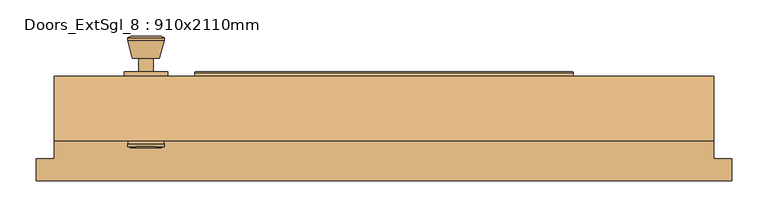
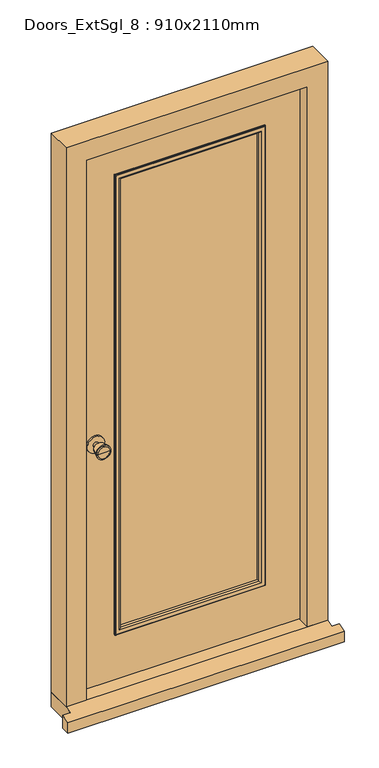
"""IFC4 building model written with IfcOpenShell, lengths in millimetres: door geometry, Doors_ExtSgl_8 : 910x2110mm."""

from ifc_helpers import new_model, si_unit, point, frame, frame_2d, origin, place, context, project, spatial, polyline, circle_curve, ellipse_curve, trimmed, segment, composite_curve, outline, extrude, faceted_brep, source, transform, mapped, element, save
from ifc_brep_helpers import plane_surface, cylinder_surface, revolved_surface, advanced_brep


def doors_extsgl_8_910x2110mm_7df14444(model_context):
    return source(origin(), model_context, "Body", "SolidModel", [
        advanced_brep(
        [(-328.5, -25.0, 950.0), (-338.5, -25.0, 950.0), (-318.5, -25.0, 950.0), (-308.0241324, 24.0, 950.0), (-348.9758676, 24.0, 950.0), (-328.5, 24.0, 950.0), (-303.5, 22.1721319, 950.0), (-353.5, 22.1721319, 950.0), (-303.5, 18.7084537, 950.0), (-353.5, 18.7084537, 950.0), (-309.863764, -6.0, 950.0), (-347.136236, -6.0, 950.0), (-318.5, -6.0, 950.0), (-338.5, -6.0, 950.0)],
        [
            (0, 1),
            (1, 2, circle_curve(frame((-328.5, -25.0, 950.0), z_axis=(0.0, -1.0, 0.0), x_axis=(-1.0, 0.0, 0.0)), 10.0)),
            (2, 0),
            (2, 1, circle_curve(frame((-328.5, -25.0, 950.0), z_axis=(0.0, -1.0, 0.0), x_axis=(-1.0, 0.0, 0.0)), 10.0)),
            (3, 4, circle_curve(frame((-328.5, 24.0, 950.0), z_axis=(0.0, 1.0, 0.0), x_axis=(-1.0, 0.0, 0.0)), 20.4758676)),
            (4, 5),
            (5, 3),
            (4, 3, circle_curve(frame((-328.5, 24.0, 950.0), z_axis=(0.0, 1.0, 0.0), x_axis=(-1.0, 0.0, 0.0)), 20.4758676)),
            (6, 7, circle_curve(frame((-328.5, 22.1721319, 950.0), z_axis=(0.0, 1.0, 0.0), x_axis=(-1.0, 0.0, 0.0)), 25.0)),
            (7, 4),
            (3, 6),
            (7, 6, circle_curve(frame((-328.5, 22.1721319, 950.0), z_axis=(0.0, 1.0, 0.0), x_axis=(-1.0, 0.0, 0.0)), 25.0)),
            (8, 9, circle_curve(frame((-328.5, 18.7084537, 950.0), z_axis=(0.0, 1.0, 0.0), x_axis=(-1.0, 0.0, 0.0)), 25.0)),
            (9, 7),
            (6, 8),
            (9, 8, circle_curve(frame((-328.5, 18.7084537, 950.0), z_axis=(0.0, 1.0, 0.0), x_axis=(-1.0, 0.0, 0.0)), 25.0)),
            (10, 11, circle_curve(frame((-328.5, -6.0, 950.0), z_axis=(0.0, 1.0, 0.0), x_axis=(-1.0, 0.0, 0.0)), 18.636236)),
            (11, 9),
            (8, 10),
            (11, 10, circle_curve(frame((-328.5, -6.0, 950.0), z_axis=(0.0, 1.0, 0.0), x_axis=(-1.0, 0.0, 0.0)), 18.636236)),
            (12, 13, circle_curve(frame((-328.5, -6.0, 950.0), z_axis=(0.0, 1.0, 0.0), x_axis=(-1.0, 0.0, 0.0)), 10.0)),
            (13, 11),
            (10, 12),
            (13, 12, circle_curve(frame((-328.5, -6.0, 950.0), z_axis=(0.0, 1.0, 0.0), x_axis=(-1.0, 0.0, 0.0)), 10.0)),
            (1, 13),
            (12, 2),
        ],
        [
            plane_surface(frame((-328.5, -25.0, 950.0), z_axis=(0.0, -1.0, 0.0), x_axis=(-1.0, 0.0, 0.0))),
            plane_surface(frame((-328.5, 24.0, 950.0), z_axis=(0.0, 1.0, 0.0), x_axis=(-1.0, 0.0, 0.0))),
            revolved_surface(polyline([(-348.9758676, 24.0, 950.0), (-353.5, 22.1721319, 950.0)]), (-328.5, -25.0, 950.0), (0.0, -1.0, 0.0)),
            cylinder_surface(frame((-328.5, -25.0, 950.0), z_axis=(0.0, -1.0, 0.0), x_axis=(-1.0, 0.0, 0.0)), 25.0),
            revolved_surface(polyline([(-353.5, 18.7084537, 950.0), (-347.136236, -6.0, 950.0)]), (-328.5, -25.0, 950.0), (0.0, -1.0, 0.0)),
            plane_surface(frame((-328.5, -6.0, 950.0), z_axis=(0.0, -1.0, 0.0), x_axis=(-1.0, 0.0, 0.0))),
            cylinder_surface(frame((-328.5, -25.0, 950.0), z_axis=(0.0, -1.0, 0.0), x_axis=(-1.0, 0.0, 0.0)), 10.0),
        ],
        [
            (0, [[1, 2, 3]]),
            (0, [[-3, 4, -1]]),
            (1, [[5, 6, 7]]),
            (1, [[8, -7, -6]]),
            (2, [[9, 10, -5, 11]]),
            (2, [[12, -11, -8, -10]]),
            (3, [[13, 14, -9, 15]]),
            (3, [[16, -15, -12, -14]]),
            (4, [[17, 18, -13, 19]]),
            (4, [[20, -19, -16, -18]]),
            (5, [[21, 22, -17, 23]]),
            (5, [[24, -23, -20, -22]]),
            (6, [[-2, 25, -21, 26]]),
            (6, [[-4, -26, -24, -25]]),
        ],
    ),
        extrude(outline(composite_curve([segment(trimmed(circle_curve(frame_2d((950.0, -328.5)), 30.0), [point((950.0, -358.5))], [point((950.0, -298.5))], False, "CARTESIAN"), True, "CONTINUOUS"), segment(trimmed(circle_curve(frame_2d((950.0, -328.5)), 30.0), [point((950.0, -298.5))], [point((950.0, -358.5))], False, "CARTESIAN"), True, "CONTINUOUS")], self_intersect=False)), frame((0.0, -31.0, 0.0), z_axis=(0.0, 1.0, 0.0), x_axis=(0.0, 0.0, 1.0)), (0.0, 0.0, 1.0), 6.0),
        advanced_brep(
        [(-328.5, -81.0, 950.0), (-318.5, -81.0, 950.0), (-338.5, -81.0, 950.0), (-308.0241324, -130.0, 950.0), (-328.5, -130.0, 950.0), (-348.9758676, -130.0, 950.0), (-303.5, -128.1721319, 950.0), (-353.5, -128.1721319, 950.0), (-303.5, -124.7084537, 950.0), (-353.5, -124.7084537, 950.0), (-309.863764, -100.0, 950.0), (-347.136236, -100.0, 950.0), (-318.5, -100.0, 950.0), (-338.5, -100.0, 950.0)],
        [
            (0, 1),
            (1, 2, circle_curve(frame((-328.5, -81.0, 950.0), z_axis=(0.0, 1.0, 0.0), x_axis=(-1.0, 0.0, 0.0)), 10.0)),
            (2, 0),
            (2, 1, circle_curve(frame((-328.5, -81.0, 950.0), z_axis=(0.0, 1.0, 0.0), x_axis=(-1.0, 0.0, 0.0)), 10.0)),
            (3, 4),
            (4, 5),
            (5, 3, circle_curve(frame((-328.5, -130.0, 950.0), z_axis=(0.0, -1.0, 0.0), x_axis=(-1.0, 0.0, 0.0)), 20.4758676)),
            (3, 5, circle_curve(frame((-328.5, -130.0, 950.0), z_axis=(0.0, -1.0, 0.0), x_axis=(-1.0, 0.0, 0.0)), 20.4758676)),
            (6, 3),
            (5, 7),
            (7, 6, circle_curve(frame((-328.5, -128.1721319, 950.0), z_axis=(0.0, -1.0, 0.0), x_axis=(-1.0, 0.0, 0.0)), 25.0)),
            (6, 7, circle_curve(frame((-328.5, -128.1721319, 950.0), z_axis=(0.0, -1.0, 0.0), x_axis=(-1.0, 0.0, 0.0)), 25.0)),
            (8, 6),
            (7, 9),
            (9, 8, circle_curve(frame((-328.5, -124.7084537, 950.0), z_axis=(0.0, -1.0, 0.0), x_axis=(-1.0, 0.0, 0.0)), 25.0)),
            (8, 9, circle_curve(frame((-328.5, -124.7084537, 950.0), z_axis=(0.0, -1.0, 0.0), x_axis=(-1.0, 0.0, 0.0)), 25.0)),
            (10, 8),
            (9, 11),
            (11, 10, circle_curve(frame((-328.5, -100.0, 950.0), z_axis=(0.0, -1.0, 0.0), x_axis=(-1.0, 0.0, 0.0)), 18.636236)),
            (10, 11, circle_curve(frame((-328.5, -100.0, 950.0), z_axis=(0.0, -1.0, 0.0), x_axis=(-1.0, 0.0, 0.0)), 18.636236)),
            (12, 10),
            (11, 13),
            (13, 12, circle_curve(frame((-328.5, -100.0, 950.0), z_axis=(0.0, -1.0, 0.0), x_axis=(-1.0, 0.0, 0.0)), 10.0)),
            (12, 13, circle_curve(frame((-328.5, -100.0, 950.0), z_axis=(0.0, -1.0, 0.0), x_axis=(-1.0, 0.0, 0.0)), 10.0)),
            (1, 12),
            (13, 2),
        ],
        [
            plane_surface(frame((-328.5, -81.0, 950.0), z_axis=(0.0, 1.0, 0.0), x_axis=(-1.0, 0.0, 0.0))),
            plane_surface(frame((-328.5, -130.0, 950.0), z_axis=(0.0, -1.0, 0.0), x_axis=(-1.0, 0.0, 0.0))),
            revolved_surface(polyline([(-348.9758676, -130.0, 950.0), (-353.5, -128.1721319, 950.0)]), (-328.5, -81.0, 950.0), (0.0, 1.0, 0.0)),
            cylinder_surface(frame((-328.5, -81.0, 950.0), z_axis=(0.0, 1.0, 0.0), x_axis=(-1.0, 0.0, 0.0)), 25.0),
            revolved_surface(polyline([(-353.5, -124.7084537, 950.0), (-347.136236, -100.0, 950.0)]), (-328.5, -81.0, 950.0), (0.0, 1.0, 0.0)),
            plane_surface(frame((-328.5, -100.0, 950.0), z_axis=(0.0, 1.0, 0.0), x_axis=(-1.0, 0.0, 0.0))),
            cylinder_surface(frame((-328.5, -81.0, 950.0), z_axis=(0.0, 1.0, 0.0), x_axis=(-1.0, 0.0, 0.0)), 10.0),
        ],
        [
            (0, [[1, 2, 3]]),
            (0, [[-3, 4, -1]]),
            (1, [[5, 6, 7]]),
            (1, [[-6, -5, 8]]),
            (2, [[9, -7, 10, 11]]),
            (2, [[-10, -8, -9, 12]]),
            (3, [[13, -11, 14, 15]]),
            (3, [[-14, -12, -13, 16]]),
            (4, [[17, -15, 18, 19]]),
            (4, [[-18, -16, -17, 20]]),
            (5, [[21, -19, 22, 23]]),
            (5, [[-22, -20, -21, 24]]),
            (6, [[25, -23, 26, -2]]),
            (6, [[-26, -24, -25, -4]]),
        ],
    ),
        extrude(outline(composite_curve([segment(trimmed(circle_curve(frame_2d((950.0, -328.5)), 30.0), [point((950.0, -358.5))], [point((950.0, -298.5))], False, "CARTESIAN"), True, "CONTINUOUS"), segment(trimmed(circle_curve(frame_2d((950.0, -328.5)), 30.0), [point((950.0, -298.5))], [point((950.0, -358.5))], False, "CARTESIAN"), True, "CONTINUOUS")], self_intersect=False)), frame((0.0, -81.0, 0.0), z_axis=(0.0, 1.0, 0.0), x_axis=(0.0, 0.0, 1.0)), (0.0, 0.0, 1.0), 6.0),
        faceted_brep([(384.5, -120.0, 54.5), (384.5, -78.0, 54.5), (406.5, -78.0, 54.5), (406.5, -31.0, 54.5), (455.0, -31.0, 54.5), (455.0, -120.0, 54.5), (455.0, -120.0, 2110.0), (-455.0, -120.0, 2110.0), (-455.0, -120.0, 54.5), (-384.5, -120.0, 54.5), (-384.5, -120.0, 2039.5), (384.5, -120.0, 2039.5), (455.0, -31.0, 2110.0), (406.5, -31.0, 2061.5), (-406.5, -31.0, 2061.5), (-406.5, -31.0, 54.5), (-455.0, -31.0, 54.5), (-455.0, -31.0, 2110.0), (406.5, -78.0, 2061.5), (384.5, -78.0, 2039.5), (-384.5, -78.0, 2039.5), (-384.5, -78.0, 54.5), (-406.5, -78.0, 54.5), (-406.5, -78.0, 2061.5)], [[[0, 1, 2, 3, 4, 5]], [[5, 6, 7, 8, 9, 10, 11, 0]], [[4, 12, 6, 5]], [[3, 13, 14, 15, 16, 17, 12, 4]], [[2, 18, 13, 3]], [[1, 19, 20, 21, 22, 23, 18, 2]], [[0, 11, 19, 1]], [[10, 9, 21, 20]], [[9, 8, 16, 15, 22, 21]], [[17, 16, 8, 7]], [[23, 22, 15, 14]], [[12, 17, 7, 6]], [[18, 23, 14, 13]], [[11, 10, 20, 19]]]),
        extrude(outline(polyline([(253.5, -41.0), (253.5, -65.0), (-253.5, -65.0), (-253.5, -41.0), (253.5, -41.0)])), frame((0.0, 0.0, 233.5), z_axis=(0.0, 0.0, 1.0), x_axis=(1.0, 0.0, 0.0)), (0.0, 0.0, 1.0), 1675.0),
        faceted_brep([(480.0, -175.0, 0.0), (480.0, -145.0, 0.0), (480.0, -145.0, 47.2703282), (480.0, -175.0, 38.5947221), (-480.0, -175.0, 38.5947221), (-480.0, -145.0, 47.2703282), (-480.0, -145.0, 0.0), (-480.0, -175.0, 0.0), (-455.0, -145.0, 0.0), (-455.0, -31.0, 0.0), (455.0, -31.0, 0.0), (455.0, -145.0, 0.0), (455.0, -145.0, 47.2703282), (455.0, -120.0, 54.5), (-455.0, -120.0, 54.5), (-455.0, -145.0, 47.2703282), (455.0, -31.0, 54.5), (-455.0, -31.0, 54.5)], [[[0, 1, 2, 3]], [[4, 5, 6, 7]], [[7, 6, 8, 9, 10, 11, 1, 0]], [[3, 4, 7, 0]], [[3, 2, 12, 13, 14, 15, 5, 4]], [[14, 13, 16, 17]], [[17, 16, 10, 9]], [[15, 14, 17, 9, 8]], [[8, 6, 5, 15]], [[11, 10, 16, 13, 12]], [[12, 2, 1, 11]]]),
        extrude(outline(polyline([(58.5, 403.5), (2058.5, 403.5), (2058.5, -404.4250294), (58.5, -404.4250294), (58.5, 403.5)]), holes=[polyline([(233.5, -253.5), (1908.5, -253.5), (1908.5, 253.5), (233.5, 253.5), (233.5, -253.5)])]), frame((0.0, -75.0, 0.0), z_axis=(0.0, 1.0, 0.0), x_axis=(0.0, 0.0, 1.0)), (0.0, 0.0, 1.0), 44.0),
        advanced_brep(
        [(261.5, -27.0, 225.5), (261.5, -27.0, 1916.5), (261.5, -31.0, 1916.5), (261.5, -31.0, 225.5), (259.5, -25.0, 227.5), (259.5, -25.0, 1914.5), (241.5, -30.0, 245.5), (241.5, -30.0, 1896.5), (246.5, -25.0, 1901.5), (246.5, -25.0, 240.5), (241.5, -41.0, 245.5), (241.5, -41.0, 1896.5), (253.5, -31.0, 233.5), (253.5, -31.0, 1908.5), (253.5, -41.0, 1908.5), (253.5, -41.0, 233.5), (-261.5, -27.0, 1916.5), (-261.5, -31.0, 1916.5), (-259.5, -25.0, 1914.5), (-241.5, -30.0, 1896.5), (-246.5, -25.0, 1901.5), (-241.5, -41.0, 1896.5), (-253.5, -31.0, 1908.5), (-253.5, -41.0, 1908.5), (-261.5, -27.0, 225.5), (-261.5, -31.0, 225.5), (-259.5, -25.0, 227.5), (-241.5, -30.0, 245.5), (-246.5, -25.0, 240.5), (-241.5, -41.0, 245.5), (-253.5, -31.0, 233.5), (-253.5, -41.0, 233.5)],
        [
            (0, 1),
            (1, 2),
            (2, 3),
            (3, 0),
            (4, 5),
            (5, 1, ellipse_curve(frame((259.5, -27.0, 1914.5), z_axis=(0.7071067811865521, 0.0, -0.7071067811865428), x_axis=(-0.7071067811865428, 0.0, -0.7071067811865521)), 2.8284271, 2.0)),
            (0, 4, ellipse_curve(frame((259.5, -27.0, 227.5), z_axis=(0.7071067811865427, 0.0, 0.7071067811865522), x_axis=(0.7071067811865521, 0.0, -0.7071067811865429)), 2.8284271, 2.0)),
            (6, 7),
            (7, 8, ellipse_curve(frame((246.5, -30.0, 1901.5), z_axis=(0.7071067811865521, 0.0, -0.7071067811865428), x_axis=(-0.7071067811865428, 0.0, -0.7071067811865521)), 7.0710678, 5.0)),
            (8, 9),
            (9, 6, ellipse_curve(frame((246.5, -30.0, 240.5), z_axis=(0.7071067811865427, 0.0, 0.7071067811865522), x_axis=(0.7071067811865521, 0.0, -0.7071067811865429)), 7.0710678, 5.0)),
            (10, 11),
            (11, 7),
            (6, 10),
            (12, 13),
            (13, 14),
            (14, 15),
            (15, 12),
            (1, 16),
            (16, 17),
            (17, 2),
            (5, 18),
            (18, 16, ellipse_curve(frame((-259.5, -27.0, 1914.5), z_axis=(0.7071067811865428, 0.0, 0.7071067811865521), x_axis=(0.7071067811865522, 0.0, -0.7071067811865428)), 2.8284271, 2.0)),
            (7, 19),
            (19, 20, ellipse_curve(frame((-246.5, -30.0, 1901.5), z_axis=(0.7071067811865428, 0.0, 0.7071067811865521), x_axis=(0.7071067811865522, 0.0, -0.7071067811865428)), 7.0710678, 5.0)),
            (20, 8),
            (11, 21),
            (21, 19),
            (13, 22),
            (22, 23),
            (23, 14),
            (16, 24),
            (24, 25),
            (25, 17),
            (18, 26),
            (26, 24, ellipse_curve(frame((-259.5, -27.0, 227.5), z_axis=(-0.7071067811865522, 0.0, 0.7071067811865428), x_axis=(0.7071067811865428, 0.0, 0.7071067811865522)), 2.8284271, 2.0)),
            (19, 27),
            (27, 28, ellipse_curve(frame((-246.5, -30.0, 240.5), z_axis=(-0.7071067811865522, 0.0, 0.7071067811865428), x_axis=(0.7071067811865428, 0.0, 0.7071067811865522)), 7.0710678, 5.0)),
            (28, 20),
            (21, 29),
            (29, 27),
            (22, 30),
            (30, 31),
            (31, 23),
            (24, 0),
            (3, 25),
            (26, 4),
            (28, 9),
            (27, 6),
            (29, 10),
            (31, 15),
            (30, 12),
        ],
        [
            plane_surface(frame((261.5, -31.0, 225.5), z_axis=(1.0, 0.0, 0.0), x_axis=(0.0, 0.0, 1.0))),
            cylinder_surface(frame((259.5, -27.0, 233.5), z_axis=(0.0, 0.0, -1.0), x_axis=(1.0, 0.0, 0.0)), 2.0),
            cylinder_surface(frame((246.5, -30.0, 233.5), z_axis=(0.0, 0.0, -1.0), x_axis=(1.0, 0.0, 0.0)), 5.0),
            plane_surface(frame((241.5, -30.0, 245.5), z_axis=(-1.0, 0.0, 0.0), x_axis=(0.0, 0.0, 1.0))),
            plane_surface(frame((253.5, -41.0, 233.5), z_axis=(1.0, 0.0, 0.0), x_axis=(0.0, 0.0, 1.0))),
            plane_surface(frame((261.5, -31.0, 1916.5), z_axis=(0.0, 0.0, 1.0), x_axis=(-1.0, 0.0, 0.0))),
            cylinder_surface(frame((253.5, -27.0, 1914.5), z_axis=(1.0, 0.0, 0.0), x_axis=(0.0, 0.0, 1.0)), 2.0),
            cylinder_surface(frame((253.5, -30.0, 1901.5), z_axis=(1.0, 0.0, 0.0), x_axis=(0.0, 0.0, 1.0)), 5.0),
            plane_surface(frame((241.5, -30.0, 1896.5), z_axis=(0.0, 0.0, -1.0), x_axis=(-1.0, 0.0, 0.0))),
            plane_surface(frame((253.5, -41.0, 1908.5), z_axis=(0.0, 0.0, 1.0), x_axis=(-1.0, 0.0, 0.0))),
            plane_surface(frame((-261.5, -31.0, 1916.5), z_axis=(-1.0, 0.0, 0.0), x_axis=(0.0, 0.0, -1.0))),
            cylinder_surface(frame((-259.5, -27.0, 1908.5), z_axis=(0.0, 0.0, 1.0), x_axis=(-1.0, 0.0, 0.0)), 2.0),
            cylinder_surface(frame((-246.5, -30.0, 1908.5), z_axis=(0.0, 0.0, 1.0), x_axis=(-1.0, 0.0, 0.0)), 5.0),
            plane_surface(frame((-241.5, -30.0, 1896.5), z_axis=(1.0, 0.0, 0.0), x_axis=(0.0, 0.0, -1.0))),
            plane_surface(frame((-253.5, -41.0, 1908.5), z_axis=(-1.0, 0.0, 0.0), x_axis=(0.0, 0.0, -1.0))),
            plane_surface(frame((-261.5, -31.0, 225.5), z_axis=(0.0, 0.0, -1.0), x_axis=(1.0, 0.0, 0.0))),
            cylinder_surface(frame((-253.5, -27.0, 227.5), z_axis=(-1.0, 0.0, 0.0), x_axis=(0.0, 0.0, -1.0)), 2.0),
            plane_surface(frame((-259.5, -25.0, 227.5), z_axis=(0.0, 1.0, 0.0), x_axis=(1.0, 0.0, 0.0))),
            cylinder_surface(frame((-253.5, -30.0, 240.5), z_axis=(-1.0, 0.0, 0.0), x_axis=(0.0, 0.0, -1.0)), 5.0),
            plane_surface(frame((-241.5, -30.0, 245.5), z_axis=(0.0, 0.0, 1.0), x_axis=(1.0, 0.0, 0.0))),
            plane_surface(frame((-241.5, -41.0, 245.5), z_axis=(0.0, -1.0, 0.0), x_axis=(1.0, 0.0, 0.0))),
            plane_surface(frame((-253.5, -41.0, 233.5), z_axis=(0.0, 0.0, -1.0), x_axis=(1.0, 0.0, 0.0))),
            plane_surface(frame((-253.5, -31.0, 233.5), z_axis=(0.0, -1.0, 0.0), x_axis=(1.0, 0.0, 0.0))),
        ],
        [
            (0, [[1, 2, 3, 4]]),
            (1, [[5, 6, -1, 7]]),
            (2, [[8, 9, 10, 11]]),
            (3, [[12, 13, -8, 14]]),
            (4, [[15, 16, 17, 18]]),
            (5, [[19, 20, 21, -2]]),
            (6, [[22, 23, -19, -6]]),
            (7, [[24, 25, 26, -9]]),
            (8, [[27, 28, -24, -13]]),
            (9, [[29, 30, 31, -16]]),
            (10, [[32, 33, 34, -20]]),
            (11, [[35, 36, -32, -23]]),
            (12, [[37, 38, 39, -25]]),
            (13, [[40, 41, -37, -28]]),
            (14, [[42, 43, 44, -30]]),
            (15, [[45, -4, 46, -33]]),
            (16, [[47, -7, -45, -36]]),
            (17, [[-5, -47, -35, -22], [-10, -26, -39, 48]]),
            (18, [[49, -11, -48, -38]]),
            (19, [[50, -14, -49, -41]]),
            (20, [[-17, -31, -44, 51], [-12, -50, -40, -27]]),
            (21, [[52, -18, -51, -43]]),
            (22, [[-3, -21, -34, -46], [-15, -52, -42, -29]]),
        ],
    ),
        advanced_brep(
        [(-261.5, -79.0, 225.5), (-261.5, -79.0, 1916.5), (-261.5, -75.0, 1916.5), (-261.5, -75.0, 225.5), (-259.5, -81.0, 227.5), (-259.5, -81.0, 1914.5), (-241.5, -76.0, 245.5), (-241.5, -76.0, 1896.5), (-246.5, -81.0, 1901.5), (-246.5, -81.0, 240.5), (-241.5, -65.0, 245.5), (-241.5, -65.0, 1896.5), (-253.5, -75.0, 233.5), (-253.5, -75.0, 1908.5), (-253.5, -65.0, 1908.5), (-253.5, -65.0, 233.5), (261.5, -79.0, 1916.5), (261.5, -75.0, 1916.5), (259.5, -81.0, 1914.5), (241.5, -76.0, 1896.5), (246.5, -81.0, 1901.5), (241.5, -65.0, 1896.5), (253.5, -75.0, 1908.5), (253.5, -65.0, 1908.5), (261.5, -79.0, 225.5), (261.5, -75.0, 225.5), (259.5, -81.0, 227.5), (241.5, -76.0, 245.5), (246.5, -81.0, 240.5), (241.5, -65.0, 245.5), (253.5, -75.0, 233.5), (253.5, -65.0, 233.5)],
        [
            (0, 1),
            (1, 2),
            (2, 3),
            (3, 0),
            (4, 5),
            (5, 1, ellipse_curve(frame((-259.5, -79.0, 1914.5), z_axis=(-0.7071067811865475, 0.0, -0.7071067811865475), x_axis=(0.7071067811865475, 0.0, -0.7071067811865476)), 2.8284271, 2.0)),
            (0, 4, ellipse_curve(frame((-259.5, -79.0, 227.5), z_axis=(-0.7071067811865475, 0.0, 0.7071067811865476), x_axis=(-0.7071067811865475, 0.0, -0.7071067811865476)), 2.8284271, 2.0)),
            (6, 7),
            (7, 8, ellipse_curve(frame((-246.5, -76.0, 1901.5), z_axis=(-0.7071067811865475, 0.0, -0.7071067811865475), x_axis=(0.7071067811865475, 0.0, -0.7071067811865476)), 7.0710678, 5.0)),
            (8, 9),
            (9, 6, ellipse_curve(frame((-246.5, -76.0, 240.5), z_axis=(-0.7071067811865475, 0.0, 0.7071067811865476), x_axis=(-0.7071067811865475, 0.0, -0.7071067811865476)), 7.0710678, 5.0)),
            (10, 11),
            (11, 7),
            (6, 10),
            (12, 13),
            (13, 14),
            (14, 15),
            (15, 12),
            (1, 16),
            (16, 17),
            (17, 2),
            (5, 18),
            (18, 16, ellipse_curve(frame((259.5, -79.0, 1914.5), z_axis=(-0.7071067811865475, 0.0, 0.7071067811865475), x_axis=(-0.7071067811865478, 0.0, -0.7071067811865474)), 2.8284271, 2.0)),
            (7, 19),
            (19, 20, ellipse_curve(frame((246.5, -76.0, 1901.5), z_axis=(-0.7071067811865475, 0.0, 0.7071067811865475), x_axis=(-0.7071067811865478, 0.0, -0.7071067811865474)), 7.0710678, 5.0)),
            (20, 8),
            (11, 21),
            (21, 19),
            (13, 22),
            (22, 23),
            (23, 14),
            (16, 24),
            (24, 25),
            (25, 17),
            (18, 26),
            (26, 24, ellipse_curve(frame((259.5, -79.0, 227.5), z_axis=(0.7071067811865476, 0.0, 0.7071067811865475), x_axis=(-0.7071067811865475, 0.0, 0.7071067811865476)), 2.8284271, 2.0)),
            (19, 27),
            (27, 28, ellipse_curve(frame((246.5, -76.0, 240.5), z_axis=(0.7071067811865476, 0.0, 0.7071067811865475), x_axis=(-0.7071067811865475, 0.0, 0.7071067811865476)), 7.0710678, 5.0)),
            (28, 20),
            (21, 29),
            (29, 27),
            (22, 30),
            (30, 31),
            (31, 23),
            (24, 0),
            (3, 25),
            (26, 4),
            (28, 9),
            (27, 6),
            (29, 10),
            (31, 15),
            (30, 12),
        ],
        [
            plane_surface(frame((-261.5, -75.0, 225.5), z_axis=(-1.0, 0.0, 0.0), x_axis=(0.0, 0.0, 1.0))),
            cylinder_surface(frame((-259.5, -79.0, 233.5), z_axis=(0.0, 0.0, -1.0), x_axis=(-1.0, 0.0, 0.0)), 2.0),
            cylinder_surface(frame((-246.5, -76.0, 233.5), z_axis=(0.0, 0.0, -1.0), x_axis=(-1.0, 0.0, 0.0)), 5.0),
            plane_surface(frame((-241.5, -76.0, 245.5), z_axis=(1.0, 0.0, 0.0), x_axis=(0.0, 0.0, 1.0))),
            plane_surface(frame((-253.5, -65.0, 233.5), z_axis=(-1.0, 0.0, 0.0), x_axis=(0.0, 0.0, 1.0))),
            plane_surface(frame((-261.5, -75.0, 1916.5), z_axis=(0.0, 0.0, 1.0), x_axis=(1.0, 0.0, 0.0))),
            cylinder_surface(frame((-253.5, -79.0, 1914.5), z_axis=(-1.0, 0.0, 0.0), x_axis=(0.0, 0.0, 1.0)), 2.0),
            cylinder_surface(frame((-253.5, -76.0, 1901.5), z_axis=(-1.0, 0.0, 0.0), x_axis=(0.0, 0.0, 1.0)), 5.0),
            plane_surface(frame((-241.5, -76.0, 1896.5), z_axis=(0.0, 0.0, -1.0), x_axis=(1.0, 0.0, 0.0))),
            plane_surface(frame((-253.5, -65.0, 1908.5), z_axis=(0.0, 0.0, 1.0), x_axis=(1.0, 0.0, 0.0))),
            plane_surface(frame((261.5, -75.0, 1916.5), z_axis=(1.0, 0.0, 0.0), x_axis=(0.0, 0.0, -1.0))),
            cylinder_surface(frame((259.5, -79.0, 1908.5), z_axis=(0.0, 0.0, 1.0), x_axis=(1.0, 0.0, 0.0)), 2.0),
            cylinder_surface(frame((246.5, -76.0, 1908.5), z_axis=(0.0, 0.0, 1.0), x_axis=(1.0, 0.0, 0.0)), 5.0),
            plane_surface(frame((241.5, -76.0, 1896.5), z_axis=(-1.0, 0.0, 0.0), x_axis=(0.0, 0.0, -1.0))),
            plane_surface(frame((253.5, -65.0, 1908.5), z_axis=(1.0, 0.0, 0.0), x_axis=(0.0, 0.0, -1.0))),
            plane_surface(frame((261.5, -75.0, 225.5), z_axis=(0.0, 0.0, -1.0), x_axis=(-1.0, 0.0, 0.0))),
            cylinder_surface(frame((253.5, -79.0, 227.5), z_axis=(1.0, 0.0, 0.0), x_axis=(0.0, 0.0, -1.0)), 2.0),
            plane_surface(frame((259.5, -81.0, 227.5), z_axis=(0.0, -1.0, 0.0), x_axis=(-1.0, 0.0, 0.0))),
            cylinder_surface(frame((253.5, -76.0, 240.5), z_axis=(1.0, 0.0, 0.0), x_axis=(0.0, 0.0, -1.0)), 5.0),
            plane_surface(frame((241.5, -76.0, 245.5), z_axis=(0.0, 0.0, 1.0), x_axis=(-1.0, 0.0, 0.0))),
            plane_surface(frame((241.5, -65.0, 245.5), z_axis=(0.0, 1.0, 0.0), x_axis=(-1.0, 0.0, 0.0))),
            plane_surface(frame((253.5, -65.0, 233.5), z_axis=(0.0, 0.0, -1.0), x_axis=(-1.0, 0.0, 0.0))),
            plane_surface(frame((253.5, -75.0, 233.5), z_axis=(0.0, 1.0, 0.0), x_axis=(-1.0, 0.0, 0.0))),
        ],
        [
            (0, [[1, 2, 3, 4]]),
            (1, [[5, 6, -1, 7]]),
            (2, [[8, 9, 10, 11]]),
            (3, [[12, 13, -8, 14]]),
            (4, [[15, 16, 17, 18]]),
            (5, [[19, 20, 21, -2]]),
            (6, [[22, 23, -19, -6]]),
            (7, [[24, 25, 26, -9]]),
            (8, [[27, 28, -24, -13]]),
            (9, [[29, 30, 31, -16]]),
            (10, [[32, 33, 34, -20]]),
            (11, [[35, 36, -32, -23]]),
            (12, [[37, 38, 39, -25]]),
            (13, [[40, 41, -37, -28]]),
            (14, [[42, 43, 44, -30]]),
            (15, [[45, -4, 46, -33]]),
            (16, [[47, -7, -45, -36]]),
            (17, [[-5, -47, -35, -22], [-10, -26, -39, 48]]),
            (18, [[49, -11, -48, -38]]),
            (19, [[50, -14, -49, -41]]),
            (20, [[-17, -31, -44, 51], [-12, -50, -40, -27]]),
            (21, [[52, -18, -51, -43]]),
            (22, [[-3, -21, -34, -46], [-15, -52, -42, -29]]),
        ],
    ),
        extrude(outline(polyline([(253.5, -49.0), (253.5, -57.0), (-253.5, -57.0), (-253.5, -49.0), (253.5, -49.0)])), frame((0.0, 0.0, 1479.75), z_axis=(0.0, 0.0, 1.0), x_axis=(1.0, 0.0, 0.0)), (0.0, 0.0, 1.0), 20.0),
        extrude(outline(polyline([(253.5, -49.0), (253.5, -57.0), (-253.5, -57.0), (-253.5, -49.0), (253.5, -49.0)])), frame((0.0, 0.0, 1061.0), z_axis=(0.0, 0.0, 1.0), x_axis=(1.0, 0.0, 0.0)), (0.0, 0.0, 1.0), 20.0),
        extrude(outline(polyline([(253.5, -49.0), (253.5, -57.0), (-253.5, -57.0), (-253.5, -49.0), (253.5, -49.0)])), frame((0.0, 0.0, 642.25), z_axis=(0.0, 0.0, 1.0), x_axis=(1.0, 0.0, 0.0)), (0.0, 0.0, 1.0), 20.0),
    ])


if __name__ == "__main__":
    model = new_model("IFC4")
    model_context = context("Model", 3, world=origin())
    ifc_project = project(units=[si_unit("LENGTHUNIT", "METRE", prefix="MILLI")], contexts=[model_context])
    site = spatial("IfcSite", under=ifc_project)
    building = spatial("IfcBuilding", under=site)
    placement = place(None, origin())
    doors_extsgl_8_910x2110mm_shape = doors_extsgl_8_910x2110mm_7df14444(model_context)
    element("IfcDoor", 1, ObjectType="Doors_ExtSgl_8 : 910x2110mm", at=placement, inside=building, context=model_context, shape_type="MappedRepresentation", body=[
        mapped(doors_extsgl_8_910x2110mm_shape, transform((0.0, 0.0, 0.0), x_axis=(1.0, 0.0, 0.0), y_axis=(0.0, 1.0, 0.0), z_axis=(0.0, 0.0, 1.0))),
    ])
    save(model, "model.ifc")

# Revit data of these elements
# Type "Doors_ExtSgl_8 : 910x2110mm"
#   Type Mark = "55"
#   Type Comments = "External Single"
#   Operation = "SingleSwingRight"
#   Construction Type Id = "SGL"
#   Keynote = "L20"
#   Analytic Construction = "Large single-glazed windows"
#   Wrap Layers (Ext) from Ext = 102.5 mm
#   Wrap Layers (Int) from Ext = 177.5 mm
#   Visual Light Transmittance = 0.9
#   Thickness = 44 mm
#   Stile Top Rail = 150 mm
#   Stile Shutting = 150 mm
#   Stile Hanging = 150 mm
#   Stile Bottom Rail = 175 mm
#   Solar Heat Gain Coefficient = 0.86
#   Rough Width = 910 mm
#   Rough Height = 2110 mm
#   O/A Frame Width = 64 mm
#   Heat Transfer Coefficient (U) = 5.5617 W/(m²·K)
#   Handle Z Distance = 950 mm
#   Glazing Thickness = 24 mm
#   Glazing Bar Thickness = 20 mm
#   FrameWidth = 42 mm
#   FrameOffset - External = 25 mm
#   FrameDepth = 89 mm
#   Door Panel Width = 807 mm
#   Door Panel Thickness = 44 mm
#   Door Panel Height = 2000 mm
#   Cill Thickness = 54.5 mm
#   Cill Projection = 30 mm
#   Handle X Distance = 75 mm
#   Height = 2110 mm
#   Structural Tolerance = 6.5 mm
#   Tolerance = 3 mm
#   Undercut = 4 mm
#   Width = 910 mm
#   Cill Extension = 25 mm
#   Cavity Closer Width = 50 mm
#   Cavity Closer Offset from Ext = 102.5 mm
#   Cavity Closer Depth = 85 mm
#   Vis - Ironmongery = yes
#   Vis - Glazing Bars = yes
#   Vis - Cavity Closers = yes
#   Function = 1
#   Material Glazing Bars = Door - Glazing Bars
#   Material Glass = Door - Glazing
#   Material Door = Door - Panel
#   Material Frame = Door - Frame/Mullion
#   Material Ironmongery = Door - Handle
#   Wall Closure = (empty or 0)
# Element 1 (IfcDoor, "Doors_ExtSgl_8 : 910x2110mm")
#   Materials on its faces: "Door - Panel", "Door - Handle", "Door - Frame/Mullion", "Door - Glazing Bars", "Door - Glazing"
# Materials
#   "Door - Glazing Bars": class "Miscellaneous", colour RGB 158 107 65, transparency 0
#   "Door - Glazing": class "Miscellaneous", colour RGB 0 0 255, transparency 0.75
#   "Door - Panel": class "Wood", colour RGB 210 159 95, transparency 0, Keynote = "L20", Cost = 0
#   "Door - Frame/Mullion": class "Wood", colour RGB 212 179 113, transparency 0, Keynote = "L20", Cost = 0
#   "Door - Handle": class "Miscellaneous", colour RGB 0 0 0, transparency 0, Keynote = "P21", Cost = 0
